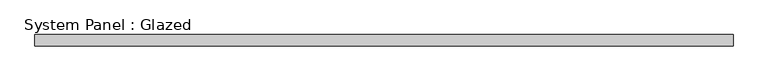
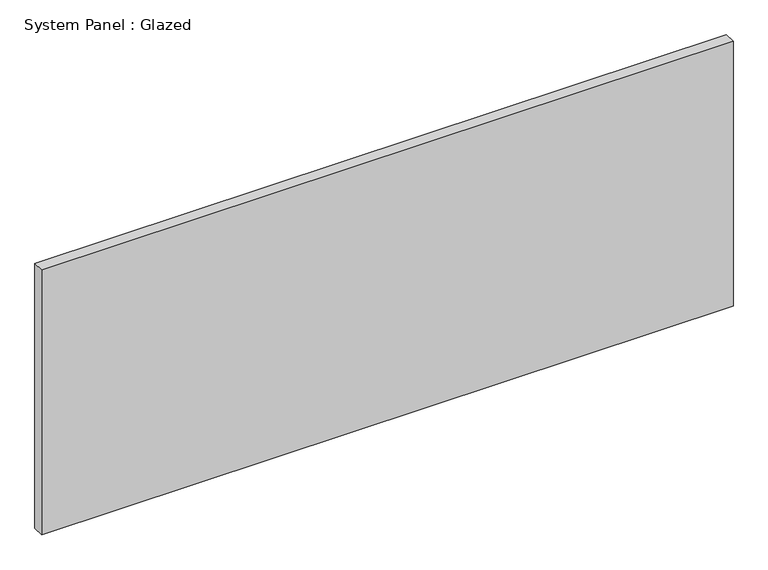
"""IFC4 building model written with IfcOpenShell, lengths in millimetres: plate geometry, System Panel : Glazed."""

import ifcopenshell
import ifcopenshell.guid

model = None  # the IFC model being written
_history = None  # IfcOwnerHistory: only IFC2X3 demands one
_inside = {}  # id of a spatial element -> (the spatial element, [elements in it])
_under = {}  # id of a project, library or spatial element -> (it, [spatial elements below it])
_declared = {}  # id of a project -> (the project, [libraries it declares])
_typed = {}  # id of a type object -> (the type object, [elements of that type])
_made_of = {}  # id of a material, layer set ... -> (it, [elements and type objects made of it])


def new_model(schema):
    """Start an empty IFC model of exactly this schema.

    Asked for "IFC4X3", IfcOpenShell would pick the latest addendum, in which some entities
    have other attributes; the version numbers below select the first issue.
    IFC2X3 requires an IfcOwnerHistory on every rooted entity: one is made here for all.
    """
    global model, _history
    if schema == "IFC4X3":
        model = ifcopenshell.file(schema_version=(4, 3, 0, 0))
    else:
        model = ifcopenshell.file(schema=schema)
    _inside.clear()
    _under.clear()
    _declared.clear()
    _typed.clear()
    _made_of.clear()
    _history = None
    if model.schema == "IFC2X3":
        org = make("IfcOrganization", Name="unknown")
        user = make(
            "IfcPersonAndOrganization",
            ThePerson=make("IfcPerson", FamilyName="unknown"),
            TheOrganization=org,
        )
        app = make(
            "IfcApplication",
            ApplicationDeveloper=org,
            Version="unknown",
            ApplicationFullName="unknown",
            ApplicationIdentifier="unknown",
        )
        _history = make(
            "IfcOwnerHistory",
            OwningUser=user,
            OwningApplication=app,
            ChangeAction="ADDED",
            CreationDate=0,
        )
    return model


def make(cls, **values):
    """One entity of the class cls with the attributes given. An attribute that is None is left unset."""
    return model.create_entity(
        cls, **{name: value for name, value in values.items() if value is not None}
    )


def rooted(cls, **values):
    """An entity with a GlobalId (a new one), such as an element, a storey or a relation."""
    return make(cls, GlobalId=ifcopenshell.guid.new(), OwnerHistory=_history, **values)


def si_unit(unit_type, name, prefix=None):
    """IfcSIUnit, for example si_unit("LENGTHUNIT", "METRE", prefix="MILLI")."""
    return make("IfcSIUnit", UnitType=unit_type, Prefix=prefix, Name=name)


def assignment(units):
    """IfcUnitAssignment: the units of a project."""
    return None if units is None else make("IfcUnitAssignment", Units=units)


def point(xyz):
    """IfcCartesianPoint."""
    return None if xyz is None else make("IfcCartesianPoint", Coordinates=xyz)


def direction(xyz):
    """IfcDirection."""
    return None if xyz is None else make("IfcDirection", DirectionRatios=xyz)


def frame(location, z_axis=None, x_axis=None):
    """IfcAxis2Placement3D, a coordinate frame: its origin and axes. An axis left out is left unset."""
    return make(
        "IfcAxis2Placement3D",
        Location=point(location),
        Axis=direction(z_axis),
        RefDirection=direction(x_axis),
    )


def origin():
    """The frame at (0, 0, 0) with its axes left unset."""
    return frame((0.0, 0.0, 0.0))


def origin_with_axes():
    """The frame at (0, 0, 0) with the z axis (0, 0, 1) and the x axis (1, 0, 0) written out."""
    return frame((0.0, 0.0, 0.0), z_axis=(0.0, 0.0, 1.0), x_axis=(1.0, 0.0, 0.0))


def place(relative_to, where):
    """IfcLocalPlacement: puts the frame where relative to a parent placement (None: the world)."""
    return make(
        "IfcLocalPlacement", PlacementRelTo=relative_to, RelativePlacement=where
    )


def context(
    kind, dimensions, precision=None, world=None, true_north=None, identifier=None
):
    """IfcGeometricRepresentationContext, for example the 3D "Model" context."""
    return make(
        "IfcGeometricRepresentationContext",
        ContextIdentifier=identifier,
        ContextType=kind,
        CoordinateSpaceDimension=dimensions,
        Precision=precision,
        WorldCoordinateSystem=world,
        TrueNorth=true_north,
    )


def project(units=None, contexts=None):
    """IfcProject with its units and contexts."""
    return rooted(
        "IfcProject",
        Name="project",
        RepresentationContexts=contexts,
        UnitsInContext=assignment(units),
    )


def spatial(cls, under=None, at=None, **own):
    """A site, building, storey or space (cls), placed at a placement, below another one or the project."""
    s = rooted(cls, ObjectPlacement=at, **own)
    if under is not None:
        _under.setdefault(under.id(), (under, []))[1].append(s)
    return s


def polyline(points):
    """IfcPolyline through the points."""
    return make("IfcPolyline", Points=[point(p) for p in points])


def outline(outer, holes=None, kind="AREA"):
    """IfcArbitraryClosedProfileDef: a profile drawn as a closed curve; with holes, ...WithVoids."""
    if holes is None:
        return make("IfcArbitraryClosedProfileDef", ProfileType=kind, OuterCurve=outer)
    return make(
        "IfcArbitraryProfileDefWithVoids",
        ProfileType=kind,
        OuterCurve=outer,
        InnerCurves=holes,
    )


def extrude(swept, where, along, depth):
    """IfcExtrudedAreaSolid: the profile swept, set in the frame where, extruded along a direction by depth."""
    return make(
        "IfcExtrudedAreaSolid",
        SweptArea=swept,
        Position=where,
        ExtrudedDirection=direction(along),
        Depth=depth,
    )


def shape(context_of_items, identifier, shape_type, items):
    """IfcShapeRepresentation: the items that make up one representation, for example the "Body"."""
    return make(
        "IfcShapeRepresentation",
        ContextOfItems=context_of_items,
        RepresentationIdentifier=identifier,
        RepresentationType=shape_type,
        Items=items,
    )


def source(mapping_origin, context_of_items, identifier, shape_type, items):
    """IfcRepresentationMap: a shape defined once, which mapped items show again and again."""
    return make(
        "IfcRepresentationMap",
        MappingOrigin=mapping_origin,
        MappedRepresentation=shape(context_of_items, identifier, shape_type, items),
    )


def transform(
    local_origin,
    x_axis=None,
    y_axis=None,
    z_axis=None,
    scale=None,
    scale2=None,
    scale3=None,
    uniform=True,
):
    """IfcCartesianTransformationOperator3D, or its non-uniform kind. x_axis, y_axis, z_axis: its Axis1, 2, 3."""
    if uniform:
        return make(
            "IfcCartesianTransformationOperator3D",
            Axis1=direction(x_axis),
            Axis2=direction(y_axis),
            LocalOrigin=point(local_origin),
            Scale=scale,
            Axis3=direction(z_axis),
        )
    return make(
        "IfcCartesianTransformationOperator3DnonUniform",
        Axis1=direction(x_axis),
        Axis2=direction(y_axis),
        LocalOrigin=point(local_origin),
        Scale=scale,
        Axis3=direction(z_axis),
        Scale2=scale2,
        Scale3=scale3,
    )


def mapped(mapping_source, mapping_target):
    """IfcMappedItem: shows the shape of a source again, moved by a transform."""
    return make(
        "IfcMappedItem", MappingSource=mapping_source, MappingTarget=mapping_target
    )


def made_of(thing, what):
    """Note that an element or type object is made of a material, layer set ...; save() writes the relation."""
    if what is not None:
        _made_of.setdefault(what.id(), (what, []))[1].append(thing)
    return thing


def element(
    cls,
    number,
    at=None,
    inside=None,
    cuts=None,
    type_object=None,
    material=None,
    context=None,
    identifier="Body",
    shape_type=None,
    held_by="IfcProductDefinitionShape",
    body=None,
    shapes=None,
    **own,
):
    """One element of the class cls, such as IfcWall. Its Tag is "e" and its number.

    at: its placement. inside: the storey or other place that contains it. cuts: it is an
    opening in that element (IfcRelVoidsElement). A single representation is given by context,
    identifier, shape_type and body (its items); several are given by shapes. held_by: the class
    of the entity that holds the representations. save() writes the other relations.
    """
    e = rooted(cls, Tag="e%d" % number, ObjectPlacement=at, **own)
    if body is not None:
        shapes = [shape(context, identifier, shape_type, body)]
    if shapes is not None:
        e.Representation = make(held_by, Representations=shapes)
    if inside is not None:
        _inside.setdefault(inside.id(), (inside, []))[1].append(e)
    if cuts is not None:
        rooted(
            "IfcRelVoidsElement", RelatingBuildingElement=cuts, RelatedOpeningElement=e
        )
    if type_object is not None:
        _typed.setdefault(type_object.id(), (type_object, []))[1].append(e)
    return made_of(e, material)


def aggregate(whole, parts):
    """IfcRelAggregates: a whole, such as a stair, and the parts it consists of."""
    return rooted("IfcRelAggregates", RelatingObject=whole, RelatedObjects=parts)


def save(model, path):
    """Write the relations noted so far, then the file.

    IfcRelAggregates (storeys below a building ...), IfcRelContainedInSpatialStructure (elements
    in a storey), IfcRelDefinesByType, IfcRelAssociatesMaterial and IfcRelDeclares: one each for
    every whole, place, type object, material and project.
    """
    for whole, parts in _under.values():
        aggregate(whole, parts)
    for where, things in _inside.values():
        rooted(
            "IfcRelContainedInSpatialStructure",
            RelatedElements=things,
            RelatingStructure=where,
        )
    for kind, things in _typed.values():
        rooted("IfcRelDefinesByType", RelatedObjects=things, RelatingType=kind)
    for what, things in _made_of.values():
        rooted("IfcRelAssociatesMaterial", RelatedObjects=things, RelatingMaterial=what)
    for by, libraries in _declared.values():
        rooted("IfcRelDeclares", RelatingContext=by, RelatedDefinitions=libraries)
    model.write(path)


def system_panel_glazed_bd26c80b(model_context):
    return source(origin(), model_context, "Body", "SweptSolid", [
        extrude(outline(polyline([(768.35, 19.05), (-768.35, 19.05), (-768.35, 44.45), (768.35, 44.45), (768.35, 19.05)])), origin_with_axes(), (0.0, 0.0, 1.0), 622.3),
    ])


if __name__ == "__main__":
    model = new_model("IFC4")
    model_context = context("Model", 3, world=origin())
    ifc_project = project(units=[si_unit("LENGTHUNIT", "METRE", prefix="MILLI")], contexts=[model_context])
    site = spatial("IfcSite", under=ifc_project)
    building = spatial("IfcBuilding", under=site)
    placement = place(None, origin())
    system_panel_glazed_shape = system_panel_glazed_bd26c80b(model_context)
    element("IfcPlate", 1, ObjectType="System Panel : Glazed", at=placement, inside=building, context=model_context, shape_type="MappedRepresentation", body=[
        mapped(system_panel_glazed_shape, transform((0.0, 0.0, 0.0), x_axis=(1.0, 0.0, 0.0), y_axis=(0.0, 1.0, 0.0), z_axis=(0.0, 0.0, 1.0))),
    ])
    save(model, "model.ifc")

# Revit data of these elements
# Element 1 (IfcPlate, "System Panel : Glazed")
#   Materials on its faces: "Glass"
# Materials
#   "Glass": class "Glass", colour RGB 0 128 192, transparency 0.75
